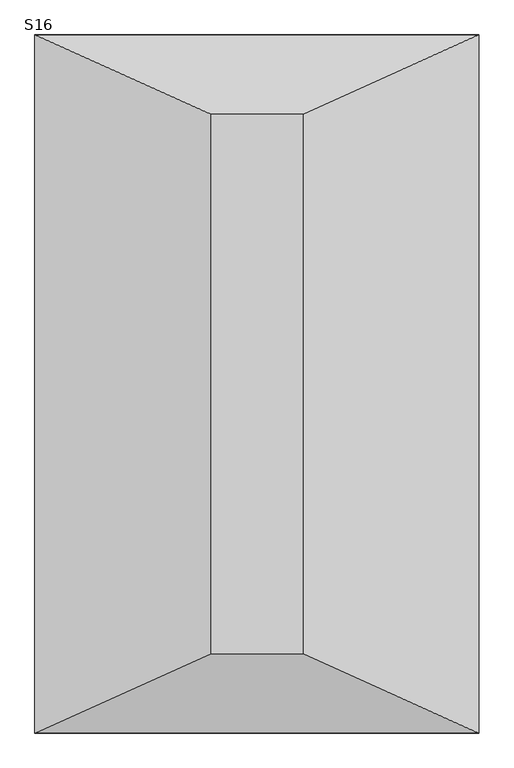
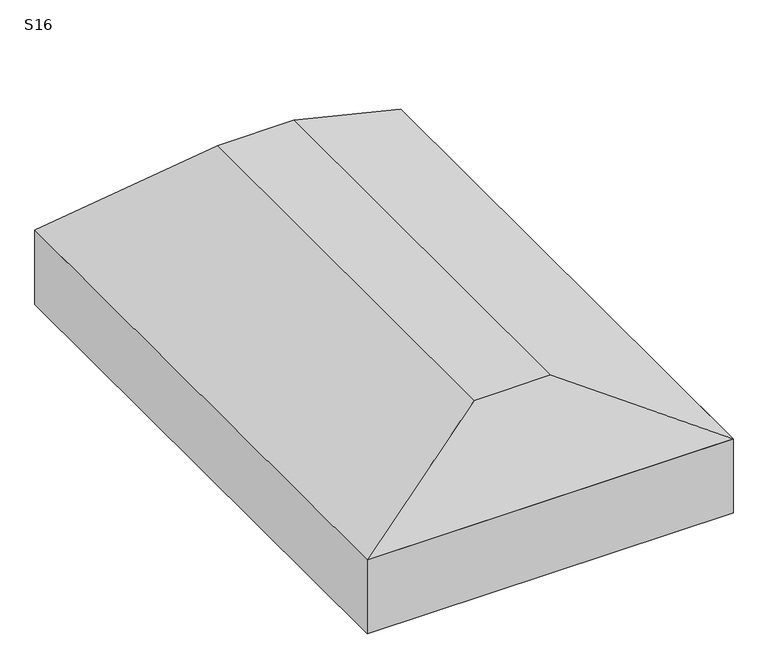
"""IFC4 building model written with IfcOpenShell, lengths in millimetres: fastener geometry, TQS - Sapata : S16."""

from ifc_helpers import new_model, si_unit, frame, origin, place, context, project, spatial, polyline, outline, extrude, faceted_brep, source, transform, mapped, element, save


def s16_25b1d231(model_context):
    return source(origin(), model_context, "Body", "SolidModel", [
        faceted_brep([(-55.0, 650.0, 0.0), (-345.0, 650.0, 0.0), (-345.0, -1050.0, 0.0), (-55.0, -1050.0, 0.0), (500.0, 900.0, -300.0), (500.0, -1300.0, -300.0), (-900.0, -1300.0, -300.0), (-900.0, 900.0, -300.0)], [[[0, 1, 2, 3]], [[4, 5, 6, 7]], [[4, 7, 1, 0]], [[7, 6, 2, 1]], [[6, 5, 3, 2]], [[5, 4, 0, 3]]]),
        extrude(outline(polyline([(500.0, 900.0), (500.0, -1300.0), (-900.0, -1300.0), (-900.0, 900.0), (500.0, 900.0)])), frame((0.0, 0.0, -600.0), z_axis=(0.0, 0.0, 1.0), x_axis=(1.0, 0.0, 0.0)), (0.0, 0.0, 1.0), 300.0),
    ])


if __name__ == "__main__":
    model = new_model("IFC4")
    model_context = context("Model", 3, world=origin())
    ifc_project = project(units=[si_unit("LENGTHUNIT", "METRE", prefix="MILLI")], contexts=[model_context])
    site = spatial("IfcSite", under=ifc_project)
    building = spatial("IfcBuilding", under=site)
    placement = place(None, origin())
    s16_shape = s16_25b1d231(model_context)
    element("IfcFastener", 1, ObjectType="TQS - Sapata : S16", at=placement, inside=building, context=model_context, shape_type="MappedRepresentation", body=[
        mapped(s16_shape, transform((0.0, 0.0, 0.0), x_axis=(1.0, 0.0, 0.0), y_axis=(0.0, 1.0, 0.0), z_axis=(0.0, 0.0, 1.0))),
    ])
    save(model, "model.ifc")

# Revit data of these elements
# Type "TQS - Sapata : S16"
#   TY = 1.70 m
#   TX = 0.29 m
#   HS = 0.60 m
#   H0 = 0.30 m
#   EXCYABS = 1.10 m
#   EXCY = 0.00 m
#   EXCXABS = 0.70 m
#   EXCX = 0.00 m
#   DIMY = 2.20 m
#   DIMX = 1.40 m
#   Material estrutural = Concreto - Concreto concretado no local
#   Width = 0
#   Length = 0
# Element 1 (IfcFastener, "TQS - Sapata : S16")
#   Materials on its faces: "Concreto - Concreto concretado no local"
# Materials
#   "Concreto - Concreto concretado no local": class "Concreto", colour RGB 192 192 192, transparency 0
